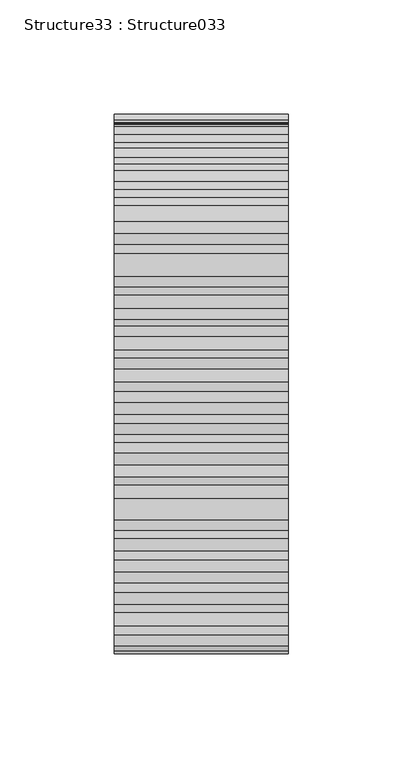
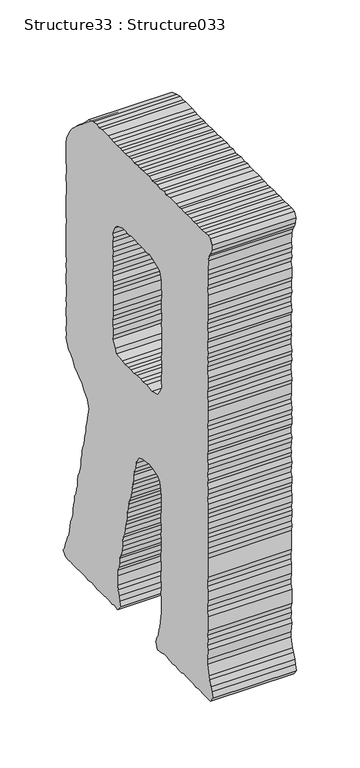
"""IFC4 building model written with IfcOpenShell, lengths in millimetres: proxy geometry, Structure33 : Structure033."""

from ifc_helpers import new_model, si_unit, frame, origin, place, context, project, spatial, polyline, outline, extrude, source, transform, mapped, element, save


def structure33_structure033_bcc766da(model_context):
    return source(origin(), model_context, "Body", "SweptSolid", [
        extrude(outline(polyline([(258948.0880727, 3899.7046941), (258948.0880727, 3894.4030808), (258948.6673349, 3890.320967), (258948.0880727, 3884.4609514), (258948.0880727, 3880.3627915), (258947.486346, 3876.263027), (258948.6673349, 3870.4030114), (258948.0880727, 3866.8776953), (258948.0880727, 3856.9179152), (258948.6673349, 3851.6612309), (258948.0880727, 3846.9757858), (258948.0880727, 3842.8583706), (258947.486346, 3838.1761347), (258948.6673349, 3832.8921721), (258947.486346, 3827.6162325), (258948.0880727, 3823.5341187), (258948.6673349, 3818.2309008), (258947.486346, 3810.0474179), (258947.486346, 3804.1890069), (258948.6673349, 3800.0876378), (258947.486346, 3794.8309535), (258948.6673349, 3790.7039107), (258948.6673349, 3785.4456218), (258947.486346, 3781.9299333), (258947.486346, 3777.2444882), (258948.6673349, 3771.3860772), (258947.486346, 3766.684586), (258948.6673349, 3762.5848215), (258944.5675704, 3753.8012165), (258940.4662013, 3751.4424479), (258937.5249613, 3747.9428055), (258934.6045811, 3743.2332913), (258930.5048166, 3739.7416719), (258927.5844364, 3737.9750024), (258923.4622075, 3734.47536), (258919.9625651, 3729.7738688), (258917.021325, 3726.2742264), (258914.1025495, 3723.9154578), (258911.7614315, 3716.2887726), (258914.1025495, 3706.9130685), (258915.2610739, 3701.0723082), (258916.4420628, 3696.9709391), (258916.4420628, 3691.6869765), (258918.202314, 3687.587212), (258919.3833029, 3683.4858429), (258919.9625651, 3678.2018803), (258921.7244208, 3674.1277895), (258922.8829453, 3670.0007467), (258923.4622075, 3665.3265338), (258924.6431964, 3660.6250426), (258924.6431964, 3654.7842823), (258927.0051742, 3646.557475), (258929.3462922, 3641.8832621), (258930.5048166, 3636.6153456), (258929.9030899, 3631.3410106), (258931.6858055, 3627.8397636), (258932.2650678, 3622.555801), (258934.6045811, 3619.0385079), (258935.2063078, 3613.772196), (258936.3664368, 3609.6547808), (258937.5249613, 3604.3964919), (258937.5249613, 3600.2967274), (258938.7059502, 3595.5872132), (258941.0454636, 3590.3289243), (258942.2264525, 3585.0706354), (258943.9883082, 3576.2693797), (258946.3278216, 3572.7440636), (258947.486346, 3568.0682461), (258949.2690616, 3564.54293), (258950.4291906, 3559.2669905), (258952.768704, 3556.3417965), (258949.2690616, 3551.6675836), (258944.5675704, 3551.0658569), (258941.0454636, 3551.6675836), (258936.3664368, 3551.0658569), (258931.0840788, 3551.0658569), (258926.4034475, 3551.6675836), (258917.6230517, 3551.6675836), (258913.5232872, 3550.4833855), (258907.6392026, 3551.6675836), (258904.1395602, 3551.6675836), (258899.4605334, 3550.4833855), (258893.5989132, 3551.0658569), (258880.1154216, 3551.0658569), (258876.0156572, 3550.4833855), (258871.9142881, 3551.6675836), (258867.2336568, 3550.4833855), (258862.5321656, 3556.3417965), (258864.2924167, 3560.441561), (258864.8716789, 3565.1254015), (258866.0526678, 3570.4109687), (258867.2336568, 3573.9266571), (258867.2336568, 3583.2863152), (258867.2336568, 3588.5702778), (258864.8716789, 3592.6700423), (258864.2924167, 3596.7698067), (258863.7131545, 3602.0280957), (258861.3736411, 3606.1551384), (258860.1910476, 3611.4134274), (258859.6117854, 3616.0972679), (258859.0325232, 3620.7971545), (258858.4307965, 3625.472972), (258856.0912831, 3629.5984101), (258855.5120209, 3634.856699), (258854.9102942, 3639.5405396), (258853.170903, 3644.2420307), (258851.989914, 3648.3161216), (258851.989914, 3652.4431643), (258850.8313896, 3657.7014533), (258849.6504007, 3662.3836892), (258847.8901496, 3667.0851803), (258846.7316251, 3670.5848228), (258844.9697694, 3675.8687854), (258844.3905072, 3679.9701544), (258843.2095182, 3685.2444894), (258842.0285293, 3689.3458585), (258842.0285293, 3695.2122926), (258840.8475404, 3698.711935), (258839.1097538, 3703.4134261), (258837.9271602, 3709.2718371), (258833.8273958, 3716.8985223), (258826.7847866, 3719.8140887), (258820.9456309, 3719.8140887), (258817.4251286, 3720.9726131), (258811.5635084, 3719.8140887), (258803.3623748, 3717.4729707), (258800.4419946, 3713.9556777), (258798.6817435, 3706.9130685), (258797.5007546, 3701.6547796), (258797.5007546, 3688.1873341), (258798.6817435, 3683.4858429), (258798.6817435, 3677.6274319), (258797.5007546, 3672.9435914), (258798.0800168, 3668.2437048), (258798.6817435, 3664.7440624), (258798.0800168, 3660.0682449), (258798.0800168, 3654.1841602), (258797.5007546, 3650.1004418), (258798.6817435, 3644.8245022), (258798.6817435, 3640.114988), (258798.0800168, 3636.6153456), (258797.5007546, 3631.915459), (258798.6817435, 3626.0554434), (258798.6817435, 3621.3732075), (258797.5007546, 3617.2718384), (258797.5007546, 3613.1720739), (258798.6817435, 3607.8961343), (258797.5007546, 3602.6298224), (258798.0800168, 3597.9540049), (258798.0800168, 3594.4286888), (258797.5007546, 3589.1527492), (258798.6817435, 3585.0706354), (258799.8402679, 3574.5107332), (258801.6229835, 3570.9854171), (258802.7606481, 3565.1254015), (258805.1226259, 3561.6257591), (258806.3036148, 3556.3417965), (258803.941637, 3550.4833855), (258798.0800168, 3551.0658569), (258793.3993855, 3552.242032), (258789.299621, 3552.242032), (258785.1982519, 3551.6675836), (258779.9174985, 3551.0658569), (258775.2368672, 3551.6675836), (258771.1354981, 3551.0658569), (258766.4340069, 3551.0658569), (258762.3551023, 3552.242032), (258757.6536111, 3551.6675836), (258747.7130863, 3551.6675836), (258743.0115951, 3551.0658569), (258738.910226, 3551.6675836), (258728.9488413, 3551.6675836), (258724.8474722, 3551.0658569), (258720.7477077, 3551.0658569), (258716.6463387, 3556.3417965), (258718.4065898, 3561.6257591), (258719.5667188, 3565.7094775), (258721.9062322, 3570.9854171), (258723.0872211, 3574.5107332), (258725.4491989, 3583.8864372), (258725.4491989, 3588.5702778), (258724.26821, 3597.9540049), (258725.4491989, 3602.0280957), (258724.8474722, 3607.8961343), (258725.4491989, 3612.0135494), (258724.26821, 3616.69739), (258724.26821, 3630.1824862), (258725.4491989, 3634.856699), (258725.4491989, 3639.5405396), (258724.8474722, 3645.4262289), (258724.8474722, 3654.1841602), (258725.4491989, 3658.8840468), (258725.4491989, 3663.5598643), (258724.8474722, 3668.2437048), (258724.8474722, 3686.4030139), (258724.26821, 3691.0868544), (258724.8474722, 3695.786741), (258724.26821, 3701.6547796), (258724.26821, 3706.3289925), (258724.8474722, 3709.8559132), (258724.26821, 3714.5301261), (258724.26821, 3720.4158154), (258724.8474722, 3725.0996559), (258724.8474722, 3729.1737467), (258724.26821, 3733.2991849), (258724.26821, 3738.5574738), (258725.4491989, 3742.6748889), (258724.8474722, 3747.9428055), (258724.26821, 3752.6170184), (258725.4491989, 3757.8753073), (258724.8474722, 3761.418274), (258725.4491989, 3766.1021146), (258724.8474722, 3771.9605256), (258724.26821, 3776.6427615), (258725.4491989, 3780.1616592), (258725.4491989, 3786.0280932), (258724.26821, 3789.5293402), (258724.26821, 3794.8309535), (258724.8474722, 3798.9050443), (258724.26821, 3803.5872802), (258724.8474722, 3809.4729695), (258725.4491989, 3812.9726119), (258724.8474722, 3818.2309008), (258724.8474722, 3828.2163546), (258724.26821, 3831.732043), (258724.8474722, 3836.9919366), (258725.4491989, 3841.0900965), (258725.4491989, 3846.3772683), (258724.26821, 3850.4754282), (258724.8474722, 3855.7353217), (258724.26821, 3859.8591552), (258725.4491989, 3865.7015202), (258725.4491989, 3870.4030114), (258724.8474722, 3875.0772243), (258725.4491989, 3878.5784713), (258724.8474722, 3883.2863809), (258725.4491989, 3887.9621984), (258725.4491989, 3893.822214), (258724.26821, 3897.3475301), (258724.8474722, 3903.2059411), (258725.4491989, 3906.7328618), (258725.4491989, 3911.4054701), (258724.26821, 3916.0909152), (258724.8474722, 3920.7908018), (258724.8474722, 3926.6492128), (258724.26821, 3930.1745289), (258724.26821, 3939.5325823), (258725.4491989, 3944.8165449), (258724.26821, 3949.4923624), (258724.8474722, 3954.7506513), (258724.26821, 3959.4617701), (258724.8474722, 3963.5615346), (258723.6664833, 3973.5197101), (258722.5079589, 3978.2035506), (258720.1459811, 3981.7208437), (258718.4065898, 3986.4046842), (258717.8273276, 3991.6806238), (258720.1459811, 3996.390138), (258724.8474722, 3996.9645864), (258728.9488413, 3996.9645864), (258734.8104615, 3996.390138), (258738.3309638, 3996.390138), (258743.5908573, 3996.9645864), (258747.7130863, 3996.390138), (258752.3937176, 3996.9645864), (258757.6536111, 3996.9645864), (258761.7533756, 3996.390138), (258767.0357336, 3996.9645864), (258770.5562359, 3996.390138), (258775.2368672, 3996.9645864), (258784.6189897, 3996.9645864), (258790.4806099, 3996.390138), (258794.0011122, 3997.5486624), (258799.2610057, 3996.390138), (258804.5208993, 3997.5486624), (258809.223995, 3996.9645864), (258812.7444973, 3996.390138), (258817.4251286, 3997.5486624), (258821.5248931, 3996.9645864), (258826.7847866, 3997.5486624), (258831.4878824, 3996.9645864), (258835.5876469, 3997.5486624), (258841.4492671, 3996.390138), (258846.1507583, 3996.9645864), (258849.6504007, 3996.9645864), (258855.5120209, 3996.390138), (258860.1910476, 3996.390138), (258863.1114278, 3996.9645864), (258867.812919, 3996.390138), (258873.6745392, 3996.390138), (258877.1741816, 3996.9645864), (258881.8756728, 3997.5486624), (258891.8386621, 3997.5486624), (258895.9384266, 3996.9645864), (258900.6190579, 3997.5486624), (258905.9014159, 3996.390138), (258912.9424204, 3994.0233463), (258916.4420628, 3989.9460463), (258919.9625651, 3987.0048063), (258923.4622075, 3982.8793681), (258928.1653033, 3979.9621971), (258931.0840788, 3977.6194746), (258934.0253189, 3974.1214368), (258938.126688, 3970.5768654), (258940.4662013, 3967.6789497), (258943.9883082, 3962.9774586), (258947.486346, 3955.360401), (258948.0880727, 3951.2606365), (258948.0880727, 3941.8753048), (258948.6673349, 3936.0345445), (258948.6673349, 3932.4899731), (258947.486346, 3927.8077372), (258947.486346, 3923.1319197), (258948.6673349, 3918.4480792), (258947.486346, 3907.888177), (258947.486346, 3903.2059411), (258948.0880727, 3899.7046941)]), holes=[polyline([(258820.9456309, 3794.8309535), (258826.7847866, 3794.2292268), (258830.3277534, 3794.8309535), (258836.1669091, 3794.8309535), (258841.4492671, 3793.6451507), (258846.1507583, 3794.2292268), (258849.6504007, 3794.2292268), (258855.5120209, 3793.6451507), (258859.6117854, 3794.8309535), (258868.4146457, 3795.960595), (258870.1540369, 3800.0876378), (258874.2538014, 3806.5317294), (258873.6745392, 3810.6298893), (258873.6745392, 3816.4883003), (258874.2538014, 3820.015221), (258874.2538014, 3825.2911606), (258873.6745392, 3829.374879), (258873.6745392, 3834.0474873), (258873.095277, 3839.9331766), (258873.095277, 3849.3008577), (258873.6745392, 3854.0007442), (258873.095277, 3858.1021133), (258873.095277, 3862.2018778), (258874.2538014, 3867.4601667), (258874.2538014, 3871.5599312), (258873.6745392, 3876.8438938), (258873.6745392, 3880.9452629), (258874.2538014, 3885.6210804), (258873.6745392, 3890.905043), (258874.2538014, 3895.0048075), (258874.2538014, 3900.2887701), (258873.6745392, 3904.3901392), (258874.2538014, 3908.46423), (258871.3125614, 3915.5068392), (258867.812919, 3919.0321552), (258859.0325232, 3922.5494483), (258854.3534965, 3922.5494483), (258850.8313896, 3921.3748778), (258846.1507583, 3922.5494483), (258831.4878824, 3922.5494483), (258825.6262622, 3921.9733953), (258822.1041553, 3921.3748778), (258817.4251286, 3922.5494483), (258812.7444973, 3921.3748778), (258804.5208993, 3918.4480792), (258801.0212568, 3916.0909152), (258798.6817435, 3909.0627475), (258798.6817435, 3904.9645876), (258797.5007546, 3894.4030808), (258798.6817435, 3890.320967), (258798.6817435, 3880.3627915), (258797.5007546, 3876.8438938), (258798.0800168, 3871.5599312), (258798.6817435, 3867.4601667), (258797.5007546, 3861.6178018), (258798.0800168, 3858.1021133), (258798.0800168, 3839.9331766), (258798.6817435, 3834.6588416), (258797.5007546, 3830.5574726), (258797.5007546, 3825.849563), (258798.0800168, 3820.5896694), (258798.6817435, 3816.4883003), (258798.6817435, 3811.7884138), (258798.0800168, 3805.9476534), (258801.0212568, 3800.0876378), (258803.941637, 3795.960595), (258812.7444973, 3793.6451507), (258820.9456309, 3794.8309535)])]), frame((-38594.2176606, 0.0, 0.0), z_axis=(1.0, 0.0, 0.0), x_axis=(0.0, 1.0, 0.0)), (0.0, 0.0, 1.0), 76.2),
    ])


if __name__ == "__main__":
    model = new_model("IFC4")
    model_context = context("Model", 3, world=origin())
    ifc_project = project(units=[si_unit("LENGTHUNIT", "METRE", prefix="MILLI")], contexts=[model_context])
    site = spatial("IfcSite", under=ifc_project)
    building = spatial("IfcBuilding", under=site)
    placement = place(None, origin())
    structure33_structure033_shape = structure33_structure033_bcc766da(model_context)
    element("IfcBuildingElementProxy", 1, Name="Structure33 : Structure033", ObjectType="Structure33 : Structure033", at=placement, inside=building, context=model_context, shape_type="MappedRepresentation", body=[
        mapped(structure33_structure033_shape, transform((0.0, 0.0, 0.0), x_axis=(1.0, 0.0, 0.0), y_axis=(0.0, 1.0, 0.0), z_axis=(0.0, 0.0, 1.0))),
    ])
    save(model, "model.ifc")

# Revit data of these elements
# Type "Structure33 : Structure033"
#   NameOverride = "Structure033"
# Element 1 (IfcBuildingElementProxy, "Structure33 : Structure033")
#   Materials on its faces: "BRUSHED ALUM. LETTERING"
# Materials
#   "BRUSHED ALUM. LETTERING": class "Unassigned", colour RGB 169 181 186, transparency 0, Cost = 0
